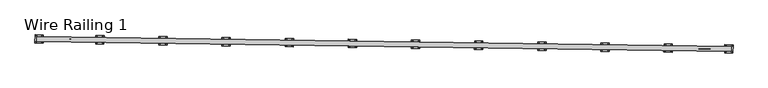
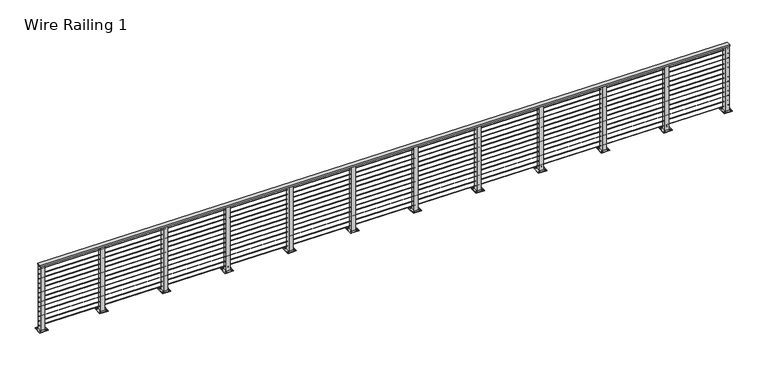
"""IFC4 building model written with IfcOpenShell, lengths in millimetres: railing geometry, Wire Railing 1."""

import ifcopenshell
import ifcopenshell.guid

model = None  # the IFC model being written
_history = None  # IfcOwnerHistory: only IFC2X3 demands one
_inside = {}  # id of a spatial element -> (the spatial element, [elements in it])
_under = {}  # id of a project, library or spatial element -> (it, [spatial elements below it])
_declared = {}  # id of a project -> (the project, [libraries it declares])
_typed = {}  # id of a type object -> (the type object, [elements of that type])
_made_of = {}  # id of a material, layer set ... -> (it, [elements and type objects made of it])


def new_model(schema):
    """Start an empty IFC model of exactly this schema.

    Asked for "IFC4X3", IfcOpenShell would pick the latest addendum, in which some entities
    have other attributes; the version numbers below select the first issue.
    IFC2X3 requires an IfcOwnerHistory on every rooted entity: one is made here for all.
    """
    global model, _history
    if schema == "IFC4X3":
        model = ifcopenshell.file(schema_version=(4, 3, 0, 0))
    else:
        model = ifcopenshell.file(schema=schema)
    _inside.clear()
    _under.clear()
    _declared.clear()
    _typed.clear()
    _made_of.clear()
    _history = None
    if model.schema == "IFC2X3":
        org = make("IfcOrganization", Name="unknown")
        user = make(
            "IfcPersonAndOrganization",
            ThePerson=make("IfcPerson", FamilyName="unknown"),
            TheOrganization=org,
        )
        app = make(
            "IfcApplication",
            ApplicationDeveloper=org,
            Version="unknown",
            ApplicationFullName="unknown",
            ApplicationIdentifier="unknown",
        )
        _history = make(
            "IfcOwnerHistory",
            OwningUser=user,
            OwningApplication=app,
            ChangeAction="ADDED",
            CreationDate=0,
        )
    return model


def make(cls, **values):
    """One entity of the class cls with the attributes given. An attribute that is None is left unset."""
    return model.create_entity(
        cls, **{name: value for name, value in values.items() if value is not None}
    )


def rooted(cls, **values):
    """An entity with a GlobalId (a new one), such as an element, a storey or a relation."""
    return make(cls, GlobalId=ifcopenshell.guid.new(), OwnerHistory=_history, **values)


def si_unit(unit_type, name, prefix=None):
    """IfcSIUnit, for example si_unit("LENGTHUNIT", "METRE", prefix="MILLI")."""
    return make("IfcSIUnit", UnitType=unit_type, Prefix=prefix, Name=name)


def assignment(units):
    """IfcUnitAssignment: the units of a project."""
    return None if units is None else make("IfcUnitAssignment", Units=units)


def point(xyz):
    """IfcCartesianPoint."""
    return None if xyz is None else make("IfcCartesianPoint", Coordinates=xyz)


def direction(xyz):
    """IfcDirection."""
    return None if xyz is None else make("IfcDirection", DirectionRatios=xyz)


def frame(location, z_axis=None, x_axis=None):
    """IfcAxis2Placement3D, a coordinate frame: its origin and axes. An axis left out is left unset."""
    return make(
        "IfcAxis2Placement3D",
        Location=point(location),
        Axis=direction(z_axis),
        RefDirection=direction(x_axis),
    )


def frame_2d(location, x_axis=None):
    """IfcAxis2Placement2D, a coordinate frame in the plane: its origin and x axis."""
    return make(
        "IfcAxis2Placement2D", Location=point(location), RefDirection=direction(x_axis)
    )


def origin():
    """The frame at (0, 0, 0) with its axes left unset."""
    return frame((0.0, 0.0, 0.0))


def place(relative_to, where):
    """IfcLocalPlacement: puts the frame where relative to a parent placement (None: the world)."""
    return make(
        "IfcLocalPlacement", PlacementRelTo=relative_to, RelativePlacement=where
    )


def context(
    kind, dimensions, precision=None, world=None, true_north=None, identifier=None
):
    """IfcGeometricRepresentationContext, for example the 3D "Model" context."""
    return make(
        "IfcGeometricRepresentationContext",
        ContextIdentifier=identifier,
        ContextType=kind,
        CoordinateSpaceDimension=dimensions,
        Precision=precision,
        WorldCoordinateSystem=world,
        TrueNorth=true_north,
    )


def project(units=None, contexts=None):
    """IfcProject with its units and contexts."""
    return rooted(
        "IfcProject",
        Name="project",
        RepresentationContexts=contexts,
        UnitsInContext=assignment(units),
    )


def spatial(cls, under=None, at=None, **own):
    """A site, building, storey or space (cls), placed at a placement, below another one or the project."""
    s = rooted(cls, ObjectPlacement=at, **own)
    if under is not None:
        _under.setdefault(under.id(), (under, []))[1].append(s)
    return s


def polyline(points):
    """IfcPolyline through the points."""
    return make("IfcPolyline", Points=[point(p) for p in points])


def circle_curve(where, radius):
    """IfcCircle in the frame where."""
    return make("IfcCircle", Position=where, Radius=radius)


def trimmed(basis, trim1, trim2, sense, master):
    """IfcTrimmedCurve: the piece of a basis curve between two trims."""
    return make(
        "IfcTrimmedCurve",
        BasisCurve=basis,
        Trim1=trim1,
        Trim2=trim2,
        SenseAgreement=sense,
        MasterRepresentation=master,
    )


def segment(curve, same_sense, transition):
    """IfcCompositeCurveSegment."""
    return make(
        "IfcCompositeCurveSegment",
        Transition=transition,
        SameSense=same_sense,
        ParentCurve=curve,
    )


def composite_curve(segments, self_intersect=None):
    """IfcCompositeCurve: segments joined end to end."""
    return make("IfcCompositeCurve", Segments=segments, SelfIntersect=self_intersect)


def outline(outer, holes=None, kind="AREA"):
    """IfcArbitraryClosedProfileDef: a profile drawn as a closed curve; with holes, ...WithVoids."""
    if holes is None:
        return make("IfcArbitraryClosedProfileDef", ProfileType=kind, OuterCurve=outer)
    return make(
        "IfcArbitraryProfileDefWithVoids",
        ProfileType=kind,
        OuterCurve=outer,
        InnerCurves=holes,
    )


def extrude(swept, where, along, depth):
    """IfcExtrudedAreaSolid: the profile swept, set in the frame where, extruded along a direction by depth."""
    return make(
        "IfcExtrudedAreaSolid",
        SweptArea=swept,
        Position=where,
        ExtrudedDirection=direction(along),
        Depth=depth,
    )


def shape(context_of_items, identifier, shape_type, items):
    """IfcShapeRepresentation: the items that make up one representation, for example the "Body"."""
    return make(
        "IfcShapeRepresentation",
        ContextOfItems=context_of_items,
        RepresentationIdentifier=identifier,
        RepresentationType=shape_type,
        Items=items,
    )


def source(mapping_origin, context_of_items, identifier, shape_type, items):
    """IfcRepresentationMap: a shape defined once, which mapped items show again and again."""
    return make(
        "IfcRepresentationMap",
        MappingOrigin=mapping_origin,
        MappedRepresentation=shape(context_of_items, identifier, shape_type, items),
    )


def transform(
    local_origin,
    x_axis=None,
    y_axis=None,
    z_axis=None,
    scale=None,
    scale2=None,
    scale3=None,
    uniform=True,
):
    """IfcCartesianTransformationOperator3D, or its non-uniform kind. x_axis, y_axis, z_axis: its Axis1, 2, 3."""
    if uniform:
        return make(
            "IfcCartesianTransformationOperator3D",
            Axis1=direction(x_axis),
            Axis2=direction(y_axis),
            LocalOrigin=point(local_origin),
            Scale=scale,
            Axis3=direction(z_axis),
        )
    return make(
        "IfcCartesianTransformationOperator3DnonUniform",
        Axis1=direction(x_axis),
        Axis2=direction(y_axis),
        LocalOrigin=point(local_origin),
        Scale=scale,
        Axis3=direction(z_axis),
        Scale2=scale2,
        Scale3=scale3,
    )


def mapped(mapping_source, mapping_target):
    """IfcMappedItem: shows the shape of a source again, moved by a transform."""
    return make(
        "IfcMappedItem", MappingSource=mapping_source, MappingTarget=mapping_target
    )


def made_of(thing, what):
    """Note that an element or type object is made of a material, layer set ...; save() writes the relation."""
    if what is not None:
        _made_of.setdefault(what.id(), (what, []))[1].append(thing)
    return thing


def element(
    cls,
    number,
    at=None,
    inside=None,
    cuts=None,
    type_object=None,
    material=None,
    context=None,
    identifier="Body",
    shape_type=None,
    held_by="IfcProductDefinitionShape",
    body=None,
    shapes=None,
    **own,
):
    """One element of the class cls, such as IfcWall. Its Tag is "e" and its number.

    at: its placement. inside: the storey or other place that contains it. cuts: it is an
    opening in that element (IfcRelVoidsElement). A single representation is given by context,
    identifier, shape_type and body (its items); several are given by shapes. held_by: the class
    of the entity that holds the representations. save() writes the other relations.
    """
    e = rooted(cls, Tag="e%d" % number, ObjectPlacement=at, **own)
    if body is not None:
        shapes = [shape(context, identifier, shape_type, body)]
    if shapes is not None:
        e.Representation = make(held_by, Representations=shapes)
    if inside is not None:
        _inside.setdefault(inside.id(), (inside, []))[1].append(e)
    if cuts is not None:
        rooted(
            "IfcRelVoidsElement", RelatingBuildingElement=cuts, RelatedOpeningElement=e
        )
    if type_object is not None:
        _typed.setdefault(type_object.id(), (type_object, []))[1].append(e)
    return made_of(e, material)


def aggregate(whole, parts):
    """IfcRelAggregates: a whole, such as a stair, and the parts it consists of."""
    return rooted("IfcRelAggregates", RelatingObject=whole, RelatedObjects=parts)


def save(model, path):
    """Write the relations noted so far, then the file.

    IfcRelAggregates (storeys below a building ...), IfcRelContainedInSpatialStructure (elements
    in a storey), IfcRelDefinesByType, IfcRelAssociatesMaterial and IfcRelDeclares: one each for
    every whole, place, type object, material and project.
    """
    for whole, parts in _under.values():
        aggregate(whole, parts)
    for where, things in _inside.values():
        rooted(
            "IfcRelContainedInSpatialStructure",
            RelatedElements=things,
            RelatingStructure=where,
        )
    for kind, things in _typed.values():
        rooted("IfcRelDefinesByType", RelatedObjects=things, RelatingType=kind)
    for what, things in _made_of.values():
        rooted("IfcRelAssociatesMaterial", RelatedObjects=things, RelatingMaterial=what)
    for by, libraries in _declared.values():
        rooted("IfcRelDeclares", RelatingContext=by, RelatedDefinitions=libraries)
    model.write(path)


def wire_railing_1_a902e167(model_context):
    return source(origin(), model_context, "Body", "SweptSolid", [
        extrude(outline(polyline([(35445.2454193, 41277.4063498), (35446.3492316, 41353.5983546), (45957.1135693, 41201.326324), (45956.009757, 41125.1343191), (35445.2454193, 41277.4063498)])), frame((0.0, 0.0, 267138.15), z_axis=(0.0, 0.0, 1.0), x_axis=(1.0, 0.0, 0.0)), (0.0, 0.0, 1.0), 19.05),
        extrude(outline(composite_curve([segment(trimmed(circle_curve(frame_2d((0.0, 2.38125)), 2.38125), [point((2.3812499, 2.38125))], [point((-2.3812501, 2.38125))], False, "CARTESIAN"), True, "CONTINUOUS"), segment(trimmed(circle_curve(frame_2d((0.0, 2.38125)), 2.38125), [point((-2.3812501, 2.38125))], [point((2.3812499, 2.38125))], False, "CARTESIAN"), True, "CONTINUOUS")], self_intersect=False)), frame((45956.5616632, 41163.2303216, 267081.0), z_axis=(-0.9998950763646337, 0.014485726138629394, 0.0), x_axis=(0.014485726138629394, 0.9998950763646337, 0.0)), (0.0, 0.0, 1.0), 10511.8672811),
        extrude(outline(composite_curve([segment(trimmed(circle_curve(frame_2d((0.0, 2.38125)), 2.38125), [point((2.3812499, 2.38125))], [point((-2.3812501, 2.38125))], False, "CARTESIAN"), True, "CONTINUOUS"), segment(trimmed(circle_curve(frame_2d((0.0, 2.38125)), 2.38125), [point((-2.3812501, 2.38125))], [point((2.3812499, 2.38125))], False, "CARTESIAN"), True, "CONTINUOUS")], self_intersect=False)), frame((45956.5616632, 41163.2303216, 267004.8), z_axis=(-0.9998950763646337, 0.014485726138629394, 0.0), x_axis=(0.014485726138629394, 0.9998950763646337, 0.0)), (0.0, 0.0, 1.0), 10511.8672811),
        extrude(outline(composite_curve([segment(trimmed(circle_curve(frame_2d((0.0, 2.38125)), 2.38125), [point((2.3812499, 2.38125))], [point((-2.3812501, 2.38125))], False, "CARTESIAN"), True, "CONTINUOUS"), segment(trimmed(circle_curve(frame_2d((0.0, 2.38125)), 2.38125), [point((-2.3812501, 2.38125))], [point((2.3812499, 2.38125))], False, "CARTESIAN"), True, "CONTINUOUS")], self_intersect=False)), frame((45956.5616632, 41163.2303216, 266928.6), z_axis=(-0.9998950763646337, 0.014485726138629394, 0.0), x_axis=(0.014485726138629394, 0.9998950763646337, 0.0)), (0.0, 0.0, 1.0), 10511.8672811),
        extrude(outline(composite_curve([segment(trimmed(circle_curve(frame_2d((0.0, 2.38125)), 2.38125), [point((2.3812499, 2.38125))], [point((-2.3812501, 2.38125))], False, "CARTESIAN"), True, "CONTINUOUS"), segment(trimmed(circle_curve(frame_2d((0.0, 2.38125)), 2.38125), [point((-2.3812501, 2.38125))], [point((2.3812499, 2.38125))], False, "CARTESIAN"), True, "CONTINUOUS")], self_intersect=False)), frame((45956.5616632, 41163.2303216, 266852.4), z_axis=(-0.9998950763646337, 0.014485726138629394, 0.0), x_axis=(0.014485726138629394, 0.9998950763646337, 0.0)), (0.0, 0.0, 1.0), 10511.8672811),
        extrude(outline(composite_curve([segment(trimmed(circle_curve(frame_2d((0.0, 2.38125)), 2.38125), [point((2.3812499, 2.38125))], [point((-2.3812501, 2.38125))], False, "CARTESIAN"), True, "CONTINUOUS"), segment(trimmed(circle_curve(frame_2d((0.0, 2.38125)), 2.38125), [point((-2.3812501, 2.38125))], [point((2.3812499, 2.38125))], False, "CARTESIAN"), True, "CONTINUOUS")], self_intersect=False)), frame((45956.5616632, 41163.2303216, 266776.2), z_axis=(-0.9998950763646337, 0.014485726138629394, 0.0), x_axis=(0.014485726138629394, 0.9998950763646337, 0.0)), (0.0, 0.0, 1.0), 10511.8672811),
        extrude(outline(composite_curve([segment(trimmed(circle_curve(frame_2d((0.0, 2.38125)), 2.38125), [point((2.3812499, 2.38125))], [point((-2.3812501, 2.38125))], False, "CARTESIAN"), True, "CONTINUOUS"), segment(trimmed(circle_curve(frame_2d((0.0, 2.38125)), 2.38125), [point((-2.3812501, 2.38125))], [point((2.3812499, 2.38125))], False, "CARTESIAN"), True, "CONTINUOUS")], self_intersect=False)), frame((45956.5616632, 41163.2303216, 266700.0), z_axis=(-0.9998950763646337, 0.014485726138629394, 0.0), x_axis=(0.014485726138629394, 0.9998950763646337, 0.0)), (0.0, 0.0, 1.0), 10511.8672811),
        extrude(outline(composite_curve([segment(trimmed(circle_curve(frame_2d((0.0, 2.38125)), 2.38125), [point((2.3812499, 2.38125))], [point((-2.3812501, 2.38125))], False, "CARTESIAN"), True, "CONTINUOUS"), segment(trimmed(circle_curve(frame_2d((0.0, 2.38125)), 2.38125), [point((-2.3812501, 2.38125))], [point((2.3812499, 2.38125))], False, "CARTESIAN"), True, "CONTINUOUS")], self_intersect=False)), frame((45956.5616632, 41163.2303216, 266623.8), z_axis=(-0.9998950763646337, 0.014485726138629394, 0.0), x_axis=(0.014485726138629394, 0.9998950763646337, 0.0)), (0.0, 0.0, 1.0), 10511.8672811),
        extrude(outline(composite_curve([segment(trimmed(circle_curve(frame_2d((0.0, 2.38125)), 2.38125), [point((2.3812499, 2.38125))], [point((-2.3812501, 2.38125))], False, "CARTESIAN"), True, "CONTINUOUS"), segment(trimmed(circle_curve(frame_2d((0.0, 2.38125)), 2.38125), [point((-2.3812501, 2.38125))], [point((2.3812499, 2.38125))], False, "CARTESIAN"), True, "CONTINUOUS")], self_intersect=False)), frame((45956.5616632, 41163.2303216, 266547.6), z_axis=(-0.9998950763646337, 0.014485726138629394, 0.0), x_axis=(0.014485726138629394, 0.9998950763646337, 0.0)), (0.0, 0.0, 1.0), 10511.8672811),
        extrude(outline(composite_curve([segment(trimmed(circle_curve(frame_2d((0.0, 2.38125)), 2.38125), [point((2.3812499, 2.38125))], [point((-2.3812501, 2.38125))], False, "CARTESIAN"), True, "CONTINUOUS"), segment(trimmed(circle_curve(frame_2d((0.0, 2.38125)), 2.38125), [point((-2.3812501, 2.38125))], [point((2.3812499, 2.38125))], False, "CARTESIAN"), True, "CONTINUOUS")], self_intersect=False)), frame((45956.5616632, 41163.2303216, 266471.4), z_axis=(-0.9998950763646337, 0.014485726138629394, 0.0), x_axis=(0.014485726138629394, 0.9998950763646337, 0.0)), (0.0, 0.0, 1.0), 10511.8672811),
        extrude(outline(composite_curve([segment(trimmed(circle_curve(frame_2d((0.0, 2.38125)), 2.38125), [point((2.3812499, 2.38125))], [point((-2.3812501, 2.38125))], False, "CARTESIAN"), True, "CONTINUOUS"), segment(trimmed(circle_curve(frame_2d((0.0, 2.38125)), 2.38125), [point((-2.3812501, 2.38125))], [point((2.3812499, 2.38125))], False, "CARTESIAN"), True, "CONTINUOUS")], self_intersect=False)), frame((45956.5616632, 41163.2303216, 266395.2), z_axis=(-0.9998950763646337, 0.014485726138629394, 0.0), x_axis=(0.014485726138629394, 0.9998950763646337, 0.0)), (0.0, 0.0, 1.0), 10511.8672811),
        extrude(outline(composite_curve([segment(trimmed(circle_curve(frame_2d((0.0, 2.38125)), 2.38125), [point((2.3812499, 2.38125))], [point((-2.3812501, 2.38125))], False, "CARTESIAN"), True, "CONTINUOUS"), segment(trimmed(circle_curve(frame_2d((0.0, 2.38125)), 2.38125), [point((-2.3812501, 2.38125))], [point((2.3812499, 2.38125))], False, "CARTESIAN"), True, "CONTINUOUS")], self_intersect=False)), frame((45956.5616632, 41163.2303216, 266319.0), z_axis=(-0.9998950763646337, 0.014485726138629394, 0.0), x_axis=(0.014485726138629394, 0.9998950763646337, 0.0)), (0.0, 0.0, 1.0), 10511.8672811),
        extrude(outline(composite_curve([segment(trimmed(circle_curve(frame_2d((0.0, 2.38125)), 2.38125), [point((2.3812499, 2.38125))], [point((-2.3812501, 2.38125))], False, "CARTESIAN"), True, "CONTINUOUS"), segment(trimmed(circle_curve(frame_2d((0.0, 2.38125)), 2.38125), [point((-2.3812501, 2.38125))], [point((2.3812499, 2.38125))], False, "CARTESIAN"), True, "CONTINUOUS")], self_intersect=False)), frame((45956.5616632, 41163.2303216, 266242.8), z_axis=(-0.9998950763646337, 0.014485726138629394, 0.0), x_axis=(0.014485726138629394, 0.9998950763646337, 0.0)), (0.0, 0.0, 1.0), 10511.8672811),
        extrude(outline(composite_curve([segment(trimmed(circle_curve(frame_2d((0.0, 2.38125)), 2.38125), [point((2.3812499, 2.38125))], [point((-2.3812501, 2.38125))], False, "CARTESIAN"), True, "CONTINUOUS"), segment(trimmed(circle_curve(frame_2d((0.0, 2.38125)), 2.38125), [point((-2.3812501, 2.38125))], [point((2.3812499, 2.38125))], False, "CARTESIAN"), True, "CONTINUOUS")], self_intersect=False)), frame((45956.5616632, 41163.2303216, 266166.6), z_axis=(-0.9998950763646337, 0.014485726138629394, 0.0), x_axis=(0.014485726138629394, 0.9998950763646337, 0.0)), (0.0, 0.0, 1.0), 10511.8672811),
        extrude(outline(composite_curve([segment(trimmed(circle_curve(frame_2d((44955.9484058, 41133.2717878)), 6.35), [point((44955.8564214, 41126.9224541))], [point((44956.0403902, 41139.6211215))], False, "CARTESIAN"), True, "CONTINUOUS"), segment(trimmed(circle_curve(frame_2d((44955.9484058, 41133.2717878)), 6.35), [point((44956.0403902, 41139.6211215))], [point((44955.8564214, 41126.9224541))], False, "CARTESIAN"), True, "CONTINUOUS")], self_intersect=False)), frame((0.0, 0.0, 266090.4), z_axis=(0.0, 0.0, 1.0), x_axis=(1.0, 0.0, 0.0)), (0.0, 0.0, 1.0), 12.7),
        extrude(outline(composite_curve([segment(trimmed(circle_curve(frame_2d((44957.2361869, 41222.1624601)), 6.35), [point((44957.1442025, 41215.8131264))], [point((44957.3281712, 41228.5117938))], False, "CARTESIAN"), True, "CONTINUOUS"), segment(trimmed(circle_curve(frame_2d((44957.2361869, 41222.1624601)), 6.35), [point((44957.3281712, 41228.5117938))], [point((44957.1442025, 41215.8131264))], False, "CARTESIAN"), True, "CONTINUOUS")], self_intersect=False)), frame((0.0, 0.0, 266090.4), z_axis=(0.0, 0.0, 1.0), x_axis=(1.0, 0.0, 0.0)), (0.0, 0.0, 1.0), 12.7),
        extrude(outline(composite_curve([segment(trimmed(circle_curve(frame_2d((45044.8390781, 41131.9840068)), 6.35), [point((45044.7470937, 41125.634673))], [point((45044.9310624, 41138.3333405))], False, "CARTESIAN"), True, "CONTINUOUS"), segment(trimmed(circle_curve(frame_2d((45044.8390781, 41131.9840068)), 6.35), [point((45044.9310624, 41138.3333405))], [point((45044.7470937, 41125.634673))], False, "CARTESIAN"), True, "CONTINUOUS")], self_intersect=False)), frame((0.0, 0.0, 266090.4), z_axis=(0.0, 0.0, 1.0), x_axis=(1.0, 0.0, 0.0)), (0.0, 0.0, 1.0), 12.7),
        extrude(outline(composite_curve([segment(trimmed(circle_curve(frame_2d((45046.1268591, 41220.874679)), 6.35), [point((45046.0348748, 41214.5253453))], [point((45046.2188435, 41227.2240128))], False, "CARTESIAN"), True, "CONTINUOUS"), segment(trimmed(circle_curve(frame_2d((45046.1268591, 41220.874679)), 6.35), [point((45046.2188435, 41227.2240128))], [point((45046.0348748, 41214.5253453))], False, "CARTESIAN"), True, "CONTINUOUS")], self_intersect=False)), frame((0.0, 0.0, 266090.4), z_axis=(0.0, 0.0, 1.0), x_axis=(1.0, 0.0, 0.0)), (0.0, 0.0, 1.0), 12.7),
        extrude(outline(polyline([(44938.4641387, 41241.4864144), (45065.4508134, 41239.6467272), (45063.6111262, 41112.6600525), (44936.6244515, 41114.4997397), (44938.4641387, 41241.4864144)])), frame((0.0, 0.0, 266090.4), z_axis=(0.0, 0.0, 1.0), x_axis=(1.0, 0.0, 0.0)), (0.0, 0.0, 1.0), 6.35),
        extrude(outline(polyline([(44971.3152229, 41207.6694944), (45031.6338934, 41206.795643), (45030.760042, 41146.4769725), (44970.4413715, 41147.3508239), (44971.3152229, 41207.6694944)]), holes=[polyline([(44977.5725723, 41201.2281763), (44976.8826896, 41153.6081733), (45024.5026926, 41152.9182906), (45025.1925753, 41200.5382936), (44977.5725723, 41201.2281763)])]), frame((0.0, 0.0, 266090.4), z_axis=(0.0, 0.0, 1.0), x_axis=(1.0, 0.0, 0.0)), (0.0, 0.0, 1.0), 1047.75),
        extrude(outline(composite_curve([segment(trimmed(circle_curve(frame_2d((44000.4243751, 41147.1146997)), 6.35), [point((44000.3323907, 41140.765366))], [point((44000.5163595, 41153.4640334))], False, "CARTESIAN"), True, "CONTINUOUS"), segment(trimmed(circle_curve(frame_2d((44000.4243751, 41147.1146997)), 6.35), [point((44000.5163595, 41153.4640334))], [point((44000.3323907, 41140.765366))], False, "CARTESIAN"), True, "CONTINUOUS")], self_intersect=False)), frame((0.0, 0.0, 266090.4), z_axis=(0.0, 0.0, 1.0), x_axis=(1.0, 0.0, 0.0)), (0.0, 0.0, 1.0), 12.7),
        extrude(outline(composite_curve([segment(trimmed(circle_curve(frame_2d((44001.7121561, 41236.005372)), 6.35), [point((44001.6201718, 41229.6560382))], [point((44001.8041405, 41242.3547057))], False, "CARTESIAN"), True, "CONTINUOUS"), segment(trimmed(circle_curve(frame_2d((44001.7121561, 41236.005372)), 6.35), [point((44001.8041405, 41242.3547057))], [point((44001.6201718, 41229.6560382))], False, "CARTESIAN"), True, "CONTINUOUS")], self_intersect=False)), frame((0.0, 0.0, 266090.4), z_axis=(0.0, 0.0, 1.0), x_axis=(1.0, 0.0, 0.0)), (0.0, 0.0, 1.0), 12.7),
        extrude(outline(composite_curve([segment(trimmed(circle_curve(frame_2d((44089.3150474, 41145.8269186)), 6.35), [point((44089.223063, 41139.4775849))], [point((44089.4070317, 41152.1762524))], False, "CARTESIAN"), True, "CONTINUOUS"), segment(trimmed(circle_curve(frame_2d((44089.3150474, 41145.8269186)), 6.35), [point((44089.4070317, 41152.1762524))], [point((44089.223063, 41139.4775849))], False, "CARTESIAN"), True, "CONTINUOUS")], self_intersect=False)), frame((0.0, 0.0, 266090.4), z_axis=(0.0, 0.0, 1.0), x_axis=(1.0, 0.0, 0.0)), (0.0, 0.0, 1.0), 12.7),
        extrude(outline(composite_curve([segment(trimmed(circle_curve(frame_2d((44090.6028284, 41234.7175909)), 6.35), [point((44090.5108441, 41228.3682572))], [point((44090.6948128, 41241.0669247))], False, "CARTESIAN"), True, "CONTINUOUS"), segment(trimmed(circle_curve(frame_2d((44090.6028284, 41234.7175909)), 6.35), [point((44090.6948128, 41241.0669247))], [point((44090.5108441, 41228.3682572))], False, "CARTESIAN"), True, "CONTINUOUS")], self_intersect=False)), frame((0.0, 0.0, 266090.4), z_axis=(0.0, 0.0, 1.0), x_axis=(1.0, 0.0, 0.0)), (0.0, 0.0, 1.0), 12.7),
        extrude(outline(polyline([(43982.940108, 41255.3293263), (44109.9267827, 41253.489639), (44108.0870955, 41126.5029643), (43981.1004208, 41128.3426516), (43982.940108, 41255.3293263)])), frame((0.0, 0.0, 266090.4), z_axis=(0.0, 0.0, 1.0), x_axis=(1.0, 0.0, 0.0)), (0.0, 0.0, 1.0), 6.35),
        extrude(outline(polyline([(44015.7911922, 41221.5124063), (44076.1098627, 41220.6385548), (44075.2360113, 41160.3198844), (44014.9173408, 41161.1937358), (44015.7911922, 41221.5124063)]), holes=[polyline([(44022.0485416, 41215.0710882), (44021.3586589, 41167.4510852), (44068.9786619, 41166.7612024), (44069.6685446, 41214.3812055), (44022.0485416, 41215.0710882)])]), frame((0.0, 0.0, 266090.4), z_axis=(0.0, 0.0, 1.0), x_axis=(1.0, 0.0, 0.0)), (0.0, 0.0, 1.0), 1047.75),
        extrude(outline(composite_curve([segment(trimmed(circle_curve(frame_2d((43044.9003444, 41160.9576116)), 6.35), [point((43044.80836, 41154.6082778))], [point((43044.9923287, 41167.3069453))], False, "CARTESIAN"), True, "CONTINUOUS"), segment(trimmed(circle_curve(frame_2d((43044.9003444, 41160.9576116)), 6.35), [point((43044.9923287, 41167.3069453))], [point((43044.80836, 41154.6082778))], False, "CARTESIAN"), True, "CONTINUOUS")], self_intersect=False)), frame((0.0, 0.0, 266090.4), z_axis=(0.0, 0.0, 1.0), x_axis=(1.0, 0.0, 0.0)), (0.0, 0.0, 1.0), 12.7),
        extrude(outline(composite_curve([segment(trimmed(circle_curve(frame_2d((43046.1881254, 41249.8482839)), 6.35), [point((43046.0961411, 41243.4989501))], [point((43046.2801098, 41256.1976176))], False, "CARTESIAN"), True, "CONTINUOUS"), segment(trimmed(circle_curve(frame_2d((43046.1881254, 41249.8482839)), 6.35), [point((43046.2801098, 41256.1976176))], [point((43046.0961411, 41243.4989501))], False, "CARTESIAN"), True, "CONTINUOUS")], self_intersect=False)), frame((0.0, 0.0, 266090.4), z_axis=(0.0, 0.0, 1.0), x_axis=(1.0, 0.0, 0.0)), (0.0, 0.0, 1.0), 12.7),
        extrude(outline(composite_curve([segment(trimmed(circle_curve(frame_2d((43133.7910167, 41159.6698305)), 6.35), [point((43133.6990323, 41153.3204968))], [point((43133.883001, 41166.0191642))], False, "CARTESIAN"), True, "CONTINUOUS"), segment(trimmed(circle_curve(frame_2d((43133.7910167, 41159.6698305)), 6.35), [point((43133.883001, 41166.0191642))], [point((43133.6990323, 41153.3204968))], False, "CARTESIAN"), True, "CONTINUOUS")], self_intersect=False)), frame((0.0, 0.0, 266090.4), z_axis=(0.0, 0.0, 1.0), x_axis=(1.0, 0.0, 0.0)), (0.0, 0.0, 1.0), 12.7),
        extrude(outline(composite_curve([segment(trimmed(circle_curve(frame_2d((43135.0787977, 41248.5605028)), 6.35), [point((43134.9868134, 41242.2111691))], [point((43135.1707821, 41254.9098365))], False, "CARTESIAN"), True, "CONTINUOUS"), segment(trimmed(circle_curve(frame_2d((43135.0787977, 41248.5605028)), 6.35), [point((43135.1707821, 41254.9098365))], [point((43134.9868134, 41242.2111691))], False, "CARTESIAN"), True, "CONTINUOUS")], self_intersect=False)), frame((0.0, 0.0, 266090.4), z_axis=(0.0, 0.0, 1.0), x_axis=(1.0, 0.0, 0.0)), (0.0, 0.0, 1.0), 12.7),
        extrude(outline(polyline([(43027.4160773, 41269.1722381), (43154.402752, 41267.3325509), (43152.5630648, 41140.3458762), (43025.5763901, 41142.1855634), (43027.4160773, 41269.1722381)])), frame((0.0, 0.0, 266090.4), z_axis=(0.0, 0.0, 1.0), x_axis=(1.0, 0.0, 0.0)), (0.0, 0.0, 1.0), 6.35),
        extrude(outline(polyline([(43060.2671615, 41235.3553181), (43120.585832, 41234.4814667), (43119.7119806, 41174.1627962), (43059.3933101, 41175.0366477), (43060.2671615, 41235.3553181)]), holes=[polyline([(43066.5245109, 41228.914), (43065.8346282, 41181.293997), (43113.4546312, 41180.6041143), (43114.1445139, 41228.2241173), (43066.5245109, 41228.914)])]), frame((0.0, 0.0, 266090.4), z_axis=(0.0, 0.0, 1.0), x_axis=(1.0, 0.0, 0.0)), (0.0, 0.0, 1.0), 1047.75),
        extrude(outline(composite_curve([segment(trimmed(circle_curve(frame_2d((42089.3763137, 41174.8005234)), 6.35), [point((42089.2843293, 41168.4511897))], [point((42089.468298, 41181.1498572))], False, "CARTESIAN"), True, "CONTINUOUS"), segment(trimmed(circle_curve(frame_2d((42089.3763137, 41174.8005234)), 6.35), [point((42089.468298, 41181.1498572))], [point((42089.2843293, 41168.4511897))], False, "CARTESIAN"), True, "CONTINUOUS")], self_intersect=False)), frame((0.0, 0.0, 266090.4), z_axis=(0.0, 0.0, 1.0), x_axis=(1.0, 0.0, 0.0)), (0.0, 0.0, 1.0), 12.7),
        extrude(outline(composite_curve([segment(trimmed(circle_curve(frame_2d((42090.6640947, 41263.6911957)), 6.35), [point((42090.5721104, 41257.341862))], [point((42090.7560791, 41270.0405295))], False, "CARTESIAN"), True, "CONTINUOUS"), segment(trimmed(circle_curve(frame_2d((42090.6640947, 41263.6911957)), 6.35), [point((42090.7560791, 41270.0405295))], [point((42090.5721104, 41257.341862))], False, "CARTESIAN"), True, "CONTINUOUS")], self_intersect=False)), frame((0.0, 0.0, 266090.4), z_axis=(0.0, 0.0, 1.0), x_axis=(1.0, 0.0, 0.0)), (0.0, 0.0, 1.0), 12.7),
        extrude(outline(composite_curve([segment(trimmed(circle_curve(frame_2d((42178.266986, 41173.5127424)), 6.35), [point((42178.1750016, 41167.1634087))], [point((42178.3589703, 41179.8620761))], False, "CARTESIAN"), True, "CONTINUOUS"), segment(trimmed(circle_curve(frame_2d((42178.266986, 41173.5127424)), 6.35), [point((42178.3589703, 41179.8620761))], [point((42178.1750016, 41167.1634087))], False, "CARTESIAN"), True, "CONTINUOUS")], self_intersect=False)), frame((0.0, 0.0, 266090.4), z_axis=(0.0, 0.0, 1.0), x_axis=(1.0, 0.0, 0.0)), (0.0, 0.0, 1.0), 12.7),
        extrude(outline(composite_curve([segment(trimmed(circle_curve(frame_2d((42179.554767, 41262.4034147)), 6.35), [point((42179.4627827, 41256.0540809))], [point((42179.6467514, 41268.7527484))], False, "CARTESIAN"), True, "CONTINUOUS"), segment(trimmed(circle_curve(frame_2d((42179.554767, 41262.4034147)), 6.35), [point((42179.6467514, 41268.7527484))], [point((42179.4627827, 41256.0540809))], False, "CARTESIAN"), True, "CONTINUOUS")], self_intersect=False)), frame((0.0, 0.0, 266090.4), z_axis=(0.0, 0.0, 1.0), x_axis=(1.0, 0.0, 0.0)), (0.0, 0.0, 1.0), 12.7),
        extrude(outline(polyline([(42071.8920466, 41283.01515), (42198.8787213, 41281.1754628), (42197.0390341, 41154.1887881), (42070.0523594, 41156.0284753), (42071.8920466, 41283.01515)])), frame((0.0, 0.0, 266090.4), z_axis=(0.0, 0.0, 1.0), x_axis=(1.0, 0.0, 0.0)), (0.0, 0.0, 1.0), 6.35),
        extrude(outline(polyline([(42104.7431308, 41249.19823), (42165.0618013, 41248.3243786), (42164.1879499, 41188.0057081), (42103.8692794, 41188.8795595), (42104.7431308, 41249.19823)]), holes=[polyline([(42111.0004802, 41242.7569119), (42110.3105975, 41195.1369089), (42157.9306005, 41194.4470262), (42158.6204832, 41242.0670292), (42111.0004802, 41242.7569119)])]), frame((0.0, 0.0, 266090.4), z_axis=(0.0, 0.0, 1.0), x_axis=(1.0, 0.0, 0.0)), (0.0, 0.0, 1.0), 1047.75),
        extrude(outline(composite_curve([segment(trimmed(circle_curve(frame_2d((41133.852283, 41188.6434353)), 6.35), [point((41133.7602986, 41182.2941016))], [point((41133.9442673, 41194.9927691))], False, "CARTESIAN"), True, "CONTINUOUS"), segment(trimmed(circle_curve(frame_2d((41133.852283, 41188.6434353)), 6.35), [point((41133.9442673, 41194.9927691))], [point((41133.7602986, 41182.2941016))], False, "CARTESIAN"), True, "CONTINUOUS")], self_intersect=False)), frame((0.0, 0.0, 266090.4), z_axis=(0.0, 0.0, 1.0), x_axis=(1.0, 0.0, 0.0)), (0.0, 0.0, 1.0), 12.7),
        extrude(outline(composite_curve([segment(trimmed(circle_curve(frame_2d((41135.140064, 41277.5341076)), 6.35), [point((41135.0480797, 41271.1847739))], [point((41135.2320484, 41283.8834413))], False, "CARTESIAN"), True, "CONTINUOUS"), segment(trimmed(circle_curve(frame_2d((41135.140064, 41277.5341076)), 6.35), [point((41135.2320484, 41283.8834413))], [point((41135.0480797, 41271.1847739))], False, "CARTESIAN"), True, "CONTINUOUS")], self_intersect=False)), frame((0.0, 0.0, 266090.4), z_axis=(0.0, 0.0, 1.0), x_axis=(1.0, 0.0, 0.0)), (0.0, 0.0, 1.0), 12.7),
        extrude(outline(composite_curve([segment(trimmed(circle_curve(frame_2d((41222.7429553, 41187.3556543)), 6.35), [point((41222.6509709, 41181.0063205))], [point((41222.8349396, 41193.704988))], False, "CARTESIAN"), True, "CONTINUOUS"), segment(trimmed(circle_curve(frame_2d((41222.7429553, 41187.3556543)), 6.35), [point((41222.8349396, 41193.704988))], [point((41222.6509709, 41181.0063205))], False, "CARTESIAN"), True, "CONTINUOUS")], self_intersect=False)), frame((0.0, 0.0, 266090.4), z_axis=(0.0, 0.0, 1.0), x_axis=(1.0, 0.0, 0.0)), (0.0, 0.0, 1.0), 12.7),
        extrude(outline(composite_curve([segment(trimmed(circle_curve(frame_2d((41224.0307363, 41276.2463266)), 6.35), [point((41223.938752, 41269.8969928))], [point((41224.1227207, 41282.5956603))], False, "CARTESIAN"), True, "CONTINUOUS"), segment(trimmed(circle_curve(frame_2d((41224.0307363, 41276.2463266)), 6.35), [point((41224.1227207, 41282.5956603))], [point((41223.938752, 41269.8969928))], False, "CARTESIAN"), True, "CONTINUOUS")], self_intersect=False)), frame((0.0, 0.0, 266090.4), z_axis=(0.0, 0.0, 1.0), x_axis=(1.0, 0.0, 0.0)), (0.0, 0.0, 1.0), 12.7),
        extrude(outline(polyline([(41116.3680159, 41296.8580619), (41243.3546906, 41295.0183747), (41241.5150034, 41168.0317), (41114.5283287, 41169.8713872), (41116.3680159, 41296.8580619)])), frame((0.0, 0.0, 266090.4), z_axis=(0.0, 0.0, 1.0), x_axis=(1.0, 0.0, 0.0)), (0.0, 0.0, 1.0), 6.35),
        extrude(outline(polyline([(41149.2191001, 41263.0411419), (41209.5377706, 41262.1672905), (41208.6639192, 41201.84862), (41148.3452487, 41202.7224714), (41149.2191001, 41263.0411419)]), holes=[polyline([(41155.4764495, 41256.5998238), (41154.7865668, 41208.9798208), (41202.4065698, 41208.2899381), (41203.0964525, 41255.9099411), (41155.4764495, 41256.5998238)])]), frame((0.0, 0.0, 266090.4), z_axis=(0.0, 0.0, 1.0), x_axis=(1.0, 0.0, 0.0)), (0.0, 0.0, 1.0), 1047.75),
        extrude(outline(composite_curve([segment(trimmed(circle_curve(frame_2d((40178.3282523, 41202.4863472)), 6.35), [point((40178.2362679, 41196.1370135))], [point((40178.4202366, 41208.8356809))], False, "CARTESIAN"), True, "CONTINUOUS"), segment(trimmed(circle_curve(frame_2d((40178.3282523, 41202.4863472)), 6.35), [point((40178.4202366, 41208.8356809))], [point((40178.2362679, 41196.1370135))], False, "CARTESIAN"), True, "CONTINUOUS")], self_intersect=False)), frame((0.0, 0.0, 266090.4), z_axis=(0.0, 0.0, 1.0), x_axis=(1.0, 0.0, 0.0)), (0.0, 0.0, 1.0), 12.7),
        extrude(outline(composite_curve([segment(trimmed(circle_curve(frame_2d((40179.6160333, 41291.3770195)), 6.35), [point((40179.524049, 41285.0276857))], [point((40179.7080177, 41297.7263532))], False, "CARTESIAN"), True, "CONTINUOUS"), segment(trimmed(circle_curve(frame_2d((40179.6160333, 41291.3770195)), 6.35), [point((40179.7080177, 41297.7263532))], [point((40179.524049, 41285.0276857))], False, "CARTESIAN"), True, "CONTINUOUS")], self_intersect=False)), frame((0.0, 0.0, 266090.4), z_axis=(0.0, 0.0, 1.0), x_axis=(1.0, 0.0, 0.0)), (0.0, 0.0, 1.0), 12.7),
        extrude(outline(composite_curve([segment(trimmed(circle_curve(frame_2d((40267.2189246, 41201.1985661)), 6.35), [point((40267.1269402, 41194.8492324))], [point((40267.3109089, 41207.5478999))], False, "CARTESIAN"), True, "CONTINUOUS"), segment(trimmed(circle_curve(frame_2d((40267.2189246, 41201.1985661)), 6.35), [point((40267.3109089, 41207.5478999))], [point((40267.1269402, 41194.8492324))], False, "CARTESIAN"), True, "CONTINUOUS")], self_intersect=False)), frame((0.0, 0.0, 266090.4), z_axis=(0.0, 0.0, 1.0), x_axis=(1.0, 0.0, 0.0)), (0.0, 0.0, 1.0), 12.7),
        extrude(outline(composite_curve([segment(trimmed(circle_curve(frame_2d((40268.5067056, 41290.0892384)), 6.35), [point((40268.4147213, 41283.7399047))], [point((40268.59869, 41296.4385722))], False, "CARTESIAN"), True, "CONTINUOUS"), segment(trimmed(circle_curve(frame_2d((40268.5067056, 41290.0892384)), 6.35), [point((40268.59869, 41296.4385722))], [point((40268.4147213, 41283.7399047))], False, "CARTESIAN"), True, "CONTINUOUS")], self_intersect=False)), frame((0.0, 0.0, 266090.4), z_axis=(0.0, 0.0, 1.0), x_axis=(1.0, 0.0, 0.0)), (0.0, 0.0, 1.0), 12.7),
        extrude(outline(polyline([(40160.8439852, 41310.7009738), (40287.8306599, 41308.8612866), (40285.9909727, 41181.8746119), (40159.004298, 41183.7142991), (40160.8439852, 41310.7009738)])), frame((0.0, 0.0, 266090.4), z_axis=(0.0, 0.0, 1.0), x_axis=(1.0, 0.0, 0.0)), (0.0, 0.0, 1.0), 6.35),
        extrude(outline(polyline([(40193.6950694, 41276.8840538), (40254.0137399, 41276.0102023), (40253.1398885, 41215.6915319), (40192.821218, 41216.5653833), (40193.6950694, 41276.8840538)]), holes=[polyline([(40199.9524188, 41270.4427357), (40199.2625361, 41222.8227327), (40246.8825391, 41222.13285), (40247.5724218, 41269.752853), (40199.9524188, 41270.4427357)])]), frame((0.0, 0.0, 266090.4), z_axis=(0.0, 0.0, 1.0), x_axis=(1.0, 0.0, 0.0)), (0.0, 0.0, 1.0), 1047.75),
        extrude(outline(composite_curve([segment(trimmed(circle_curve(frame_2d((39222.8042216, 41216.3292591)), 6.35), [point((39222.7122372, 41209.9799253))], [point((39222.8962059, 41222.6785928))], False, "CARTESIAN"), True, "CONTINUOUS"), segment(trimmed(circle_curve(frame_2d((39222.8042216, 41216.3292591)), 6.35), [point((39222.8962059, 41222.6785928))], [point((39222.7122372, 41209.9799253))], False, "CARTESIAN"), True, "CONTINUOUS")], self_intersect=False)), frame((0.0, 0.0, 266090.4), z_axis=(0.0, 0.0, 1.0), x_axis=(1.0, 0.0, 0.0)), (0.0, 0.0, 1.0), 12.7),
        extrude(outline(composite_curve([segment(trimmed(circle_curve(frame_2d((39224.0920026, 41305.2199314)), 6.35), [point((39224.0000183, 41298.8705976))], [point((39224.183987, 41311.5692651))], False, "CARTESIAN"), True, "CONTINUOUS"), segment(trimmed(circle_curve(frame_2d((39224.0920026, 41305.2199314)), 6.35), [point((39224.183987, 41311.5692651))], [point((39224.0000183, 41298.8705976))], False, "CARTESIAN"), True, "CONTINUOUS")], self_intersect=False)), frame((0.0, 0.0, 266090.4), z_axis=(0.0, 0.0, 1.0), x_axis=(1.0, 0.0, 0.0)), (0.0, 0.0, 1.0), 12.7),
        extrude(outline(composite_curve([segment(trimmed(circle_curve(frame_2d((39311.6948939, 41215.041478)), 6.35), [point((39311.6029095, 41208.6921443))], [point((39311.7868782, 41221.3908118))], False, "CARTESIAN"), True, "CONTINUOUS"), segment(trimmed(circle_curve(frame_2d((39311.6948939, 41215.041478)), 6.35), [point((39311.7868782, 41221.3908118))], [point((39311.6029095, 41208.6921443))], False, "CARTESIAN"), True, "CONTINUOUS")], self_intersect=False)), frame((0.0, 0.0, 266090.4), z_axis=(0.0, 0.0, 1.0), x_axis=(1.0, 0.0, 0.0)), (0.0, 0.0, 1.0), 12.7),
        extrude(outline(composite_curve([segment(trimmed(circle_curve(frame_2d((39312.9826749, 41303.9321503)), 6.35), [point((39312.8906905, 41297.5828166))], [point((39313.0746593, 41310.281484))], False, "CARTESIAN"), True, "CONTINUOUS"), segment(trimmed(circle_curve(frame_2d((39312.9826749, 41303.9321503)), 6.35), [point((39313.0746593, 41310.281484))], [point((39312.8906905, 41297.5828166))], False, "CARTESIAN"), True, "CONTINUOUS")], self_intersect=False)), frame((0.0, 0.0, 266090.4), z_axis=(0.0, 0.0, 1.0), x_axis=(1.0, 0.0, 0.0)), (0.0, 0.0, 1.0), 12.7),
        extrude(outline(polyline([(39205.3199545, 41324.5438856), (39332.3066292, 41322.7041984), (39330.466942, 41195.7175237), (39203.4802673, 41197.5572109), (39205.3199545, 41324.5438856)])), frame((0.0, 0.0, 266090.4), z_axis=(0.0, 0.0, 1.0), x_axis=(1.0, 0.0, 0.0)), (0.0, 0.0, 1.0), 6.35),
        extrude(outline(polyline([(39238.1710387, 41290.7269656), (39298.4897092, 41289.8531142), (39297.6158578, 41229.5344437), (39237.2971873, 41230.4082952), (39238.1710387, 41290.7269656)]), holes=[polyline([(39244.4283881, 41284.2856475), (39243.7385054, 41236.6656445), (39291.3585084, 41235.9757618), (39292.0483911, 41283.5957648), (39244.4283881, 41284.2856475)])]), frame((0.0, 0.0, 266090.4), z_axis=(0.0, 0.0, 1.0), x_axis=(1.0, 0.0, 0.0)), (0.0, 0.0, 1.0), 1047.75),
        extrude(outline(composite_curve([segment(trimmed(circle_curve(frame_2d((38267.2801909, 41230.1721709)), 6.35), [point((38267.1882065, 41223.8228372))], [point((38267.3721752, 41236.5215047))], False, "CARTESIAN"), True, "CONTINUOUS"), segment(trimmed(circle_curve(frame_2d((38267.2801909, 41230.1721709)), 6.35), [point((38267.3721752, 41236.5215047))], [point((38267.1882065, 41223.8228372))], False, "CARTESIAN"), True, "CONTINUOUS")], self_intersect=False)), frame((0.0, 0.0, 266090.4), z_axis=(0.0, 0.0, 1.0), x_axis=(1.0, 0.0, 0.0)), (0.0, 0.0, 1.0), 12.7),
        extrude(outline(composite_curve([segment(trimmed(circle_curve(frame_2d((38268.5679719, 41319.0628432)), 6.35), [point((38268.4759876, 41312.7135095))], [point((38268.6599563, 41325.412177))], False, "CARTESIAN"), True, "CONTINUOUS"), segment(trimmed(circle_curve(frame_2d((38268.5679719, 41319.0628432)), 6.35), [point((38268.6599563, 41325.412177))], [point((38268.4759876, 41312.7135095))], False, "CARTESIAN"), True, "CONTINUOUS")], self_intersect=False)), frame((0.0, 0.0, 266090.4), z_axis=(0.0, 0.0, 1.0), x_axis=(1.0, 0.0, 0.0)), (0.0, 0.0, 1.0), 12.7),
        extrude(outline(composite_curve([segment(trimmed(circle_curve(frame_2d((38356.1708632, 41228.8843899)), 6.35), [point((38356.0788788, 41222.5350562))], [point((38356.2628475, 41235.2337236))], False, "CARTESIAN"), True, "CONTINUOUS"), segment(trimmed(circle_curve(frame_2d((38356.1708632, 41228.8843899)), 6.35), [point((38356.2628475, 41235.2337236))], [point((38356.0788788, 41222.5350562))], False, "CARTESIAN"), True, "CONTINUOUS")], self_intersect=False)), frame((0.0, 0.0, 266090.4), z_axis=(0.0, 0.0, 1.0), x_axis=(1.0, 0.0, 0.0)), (0.0, 0.0, 1.0), 12.7),
        extrude(outline(composite_curve([segment(trimmed(circle_curve(frame_2d((38357.4586442, 41317.7750622)), 6.35), [point((38357.3666598, 41311.4257284))], [point((38357.5506286, 41324.1243959))], False, "CARTESIAN"), True, "CONTINUOUS"), segment(trimmed(circle_curve(frame_2d((38357.4586442, 41317.7750622)), 6.35), [point((38357.5506286, 41324.1243959))], [point((38357.3666598, 41311.4257284))], False, "CARTESIAN"), True, "CONTINUOUS")], self_intersect=False)), frame((0.0, 0.0, 266090.4), z_axis=(0.0, 0.0, 1.0), x_axis=(1.0, 0.0, 0.0)), (0.0, 0.0, 1.0), 12.7),
        extrude(outline(polyline([(38249.7959238, 41338.3867975), (38376.7825985, 41336.5471103), (38374.9429113, 41209.5604356), (38247.9562366, 41211.4001228), (38249.7959238, 41338.3867975)])), frame((0.0, 0.0, 266090.4), z_axis=(0.0, 0.0, 1.0), x_axis=(1.0, 0.0, 0.0)), (0.0, 0.0, 1.0), 6.35),
        extrude(outline(polyline([(38282.647008, 41304.5698775), (38342.9656785, 41303.6960261), (38342.0918271, 41243.3773556), (38281.7731566, 41244.251207), (38282.647008, 41304.5698775)]), holes=[polyline([(38288.9043574, 41298.1285594), (38288.2144747, 41250.5085564), (38335.8344777, 41249.8186737), (38336.5243604, 41297.4386767), (38288.9043574, 41298.1285594)])]), frame((0.0, 0.0, 266090.4), z_axis=(0.0, 0.0, 1.0), x_axis=(1.0, 0.0, 0.0)), (0.0, 0.0, 1.0), 1047.75),
        extrude(outline(composite_curve([segment(trimmed(circle_curve(frame_2d((37311.7561602, 41244.0150828)), 6.35), [point((37311.6641758, 41237.6657491))], [point((37311.8481445, 41250.3644166))], False, "CARTESIAN"), True, "CONTINUOUS"), segment(trimmed(circle_curve(frame_2d((37311.7561602, 41244.0150828)), 6.35), [point((37311.8481445, 41250.3644166))], [point((37311.6641758, 41237.6657491))], False, "CARTESIAN"), True, "CONTINUOUS")], self_intersect=False)), frame((0.0, 0.0, 266090.4), z_axis=(0.0, 0.0, 1.0), x_axis=(1.0, 0.0, 0.0)), (0.0, 0.0, 1.0), 12.7),
        extrude(outline(composite_curve([segment(trimmed(circle_curve(frame_2d((37313.0439412, 41332.9057551)), 6.35), [point((37312.9519569, 41326.5564214))], [point((37313.1359256, 41339.2550888))], False, "CARTESIAN"), True, "CONTINUOUS"), segment(trimmed(circle_curve(frame_2d((37313.0439412, 41332.9057551)), 6.35), [point((37313.1359256, 41339.2550888))], [point((37312.9519569, 41326.5564214))], False, "CARTESIAN"), True, "CONTINUOUS")], self_intersect=False)), frame((0.0, 0.0, 266090.4), z_axis=(0.0, 0.0, 1.0), x_axis=(1.0, 0.0, 0.0)), (0.0, 0.0, 1.0), 12.7),
        extrude(outline(composite_curve([segment(trimmed(circle_curve(frame_2d((37400.6468324, 41242.7273018)), 6.35), [point((37400.5548481, 41236.377968))], [point((37400.7388168, 41249.0766355))], False, "CARTESIAN"), True, "CONTINUOUS"), segment(trimmed(circle_curve(frame_2d((37400.6468324, 41242.7273018)), 6.35), [point((37400.7388168, 41249.0766355))], [point((37400.5548481, 41236.377968))], False, "CARTESIAN"), True, "CONTINUOUS")], self_intersect=False)), frame((0.0, 0.0, 266090.4), z_axis=(0.0, 0.0, 1.0), x_axis=(1.0, 0.0, 0.0)), (0.0, 0.0, 1.0), 12.7),
        extrude(outline(composite_curve([segment(trimmed(circle_curve(frame_2d((37401.9346135, 41331.6179741)), 6.35), [point((37401.8426291, 41325.2686403))], [point((37402.0265979, 41337.9673078))], False, "CARTESIAN"), True, "CONTINUOUS"), segment(trimmed(circle_curve(frame_2d((37401.9346135, 41331.6179741)), 6.35), [point((37402.0265979, 41337.9673078))], [point((37401.8426291, 41325.2686403))], False, "CARTESIAN"), True, "CONTINUOUS")], self_intersect=False)), frame((0.0, 0.0, 266090.4), z_axis=(0.0, 0.0, 1.0), x_axis=(1.0, 0.0, 0.0)), (0.0, 0.0, 1.0), 12.7),
        extrude(outline(polyline([(37294.2718931, 41352.2297094), (37421.2585678, 41350.3900222), (37419.4188806, 41223.4033475), (37292.4322059, 41225.2430347), (37294.2718931, 41352.2297094)])), frame((0.0, 0.0, 266090.4), z_axis=(0.0, 0.0, 1.0), x_axis=(1.0, 0.0, 0.0)), (0.0, 0.0, 1.0), 6.35),
        extrude(outline(polyline([(37327.1229773, 41318.4127894), (37387.4416478, 41317.538938), (37386.5677964, 41257.2202675), (37326.2491259, 41258.0941189), (37327.1229773, 41318.4127894)]), holes=[polyline([(37333.3803267, 41311.9714713), (37332.690444, 41264.3514683), (37380.310447, 41263.6615856), (37381.0003297, 41311.2815886), (37333.3803267, 41311.9714713)])]), frame((0.0, 0.0, 266090.4), z_axis=(0.0, 0.0, 1.0), x_axis=(1.0, 0.0, 0.0)), (0.0, 0.0, 1.0), 1047.75),
        extrude(outline(composite_curve([segment(trimmed(circle_curve(frame_2d((36356.2321295, 41257.8579947)), 6.35), [point((36356.1401451, 41251.508661))], [point((36356.3241138, 41264.2073284))], False, "CARTESIAN"), True, "CONTINUOUS"), segment(trimmed(circle_curve(frame_2d((36356.2321295, 41257.8579947)), 6.35), [point((36356.3241138, 41264.2073284))], [point((36356.1401451, 41251.508661))], False, "CARTESIAN"), True, "CONTINUOUS")], self_intersect=False)), frame((0.0, 0.0, 266090.4), z_axis=(0.0, 0.0, 1.0), x_axis=(1.0, 0.0, 0.0)), (0.0, 0.0, 1.0), 12.7),
        extrude(outline(composite_curve([segment(trimmed(circle_curve(frame_2d((36357.5199105, 41346.748667)), 6.35), [point((36357.4279261, 41340.3993333))], [point((36357.6118949, 41353.0980007))], False, "CARTESIAN"), True, "CONTINUOUS"), segment(trimmed(circle_curve(frame_2d((36357.5199105, 41346.748667)), 6.35), [point((36357.6118949, 41353.0980007))], [point((36357.4279261, 41340.3993333))], False, "CARTESIAN"), True, "CONTINUOUS")], self_intersect=False)), frame((0.0, 0.0, 266090.4), z_axis=(0.0, 0.0, 1.0), x_axis=(1.0, 0.0, 0.0)), (0.0, 0.0, 1.0), 12.7),
        extrude(outline(composite_curve([segment(trimmed(circle_curve(frame_2d((36445.1228017, 41256.5702136)), 6.35), [point((36445.0308174, 41250.2208799))], [point((36445.2147861, 41262.9195474))], False, "CARTESIAN"), True, "CONTINUOUS"), segment(trimmed(circle_curve(frame_2d((36445.1228017, 41256.5702136)), 6.35), [point((36445.2147861, 41262.9195474))], [point((36445.0308174, 41250.2208799))], False, "CARTESIAN"), True, "CONTINUOUS")], self_intersect=False)), frame((0.0, 0.0, 266090.4), z_axis=(0.0, 0.0, 1.0), x_axis=(1.0, 0.0, 0.0)), (0.0, 0.0, 1.0), 12.7),
        extrude(outline(composite_curve([segment(trimmed(circle_curve(frame_2d((36446.4105828, 41345.4608859)), 6.35), [point((36446.3185984, 41339.1115522))], [point((36446.5025672, 41351.8102197))], False, "CARTESIAN"), True, "CONTINUOUS"), segment(trimmed(circle_curve(frame_2d((36446.4105828, 41345.4608859)), 6.35), [point((36446.5025672, 41351.8102197))], [point((36446.3185984, 41339.1115522))], False, "CARTESIAN"), True, "CONTINUOUS")], self_intersect=False)), frame((0.0, 0.0, 266090.4), z_axis=(0.0, 0.0, 1.0), x_axis=(1.0, 0.0, 0.0)), (0.0, 0.0, 1.0), 12.7),
        extrude(outline(polyline([(36338.7478624, 41366.0726213), (36465.7345371, 41364.2329341), (36463.8948499, 41237.2462594), (36336.9081752, 41239.0859466), (36338.7478624, 41366.0726213)])), frame((0.0, 0.0, 266090.4), z_axis=(0.0, 0.0, 1.0), x_axis=(1.0, 0.0, 0.0)), (0.0, 0.0, 1.0), 6.35),
        extrude(outline(polyline([(36371.5989466, 41332.2557013), (36431.9176171, 41331.3818498), (36431.0437656, 41271.0631794), (36370.7250952, 41271.9370308), (36371.5989466, 41332.2557013)]), holes=[polyline([(36377.856296, 41325.8143832), (36377.1664133, 41278.1943802), (36424.7864163, 41277.5044975), (36425.476299, 41325.1245005), (36377.856296, 41325.8143832)])]), frame((0.0, 0.0, 266090.4), z_axis=(0.0, 0.0, 1.0), x_axis=(1.0, 0.0, 0.0)), (0.0, 0.0, 1.0), 1047.75),
        extrude(outline(composite_curve([segment(trimmed(circle_curve(frame_2d((45873.3764341, 41119.9807821)), 6.35), [point((45873.2844497, 41113.6314484))], [point((45873.4684185, 41126.3301158))], False, "CARTESIAN"), True, "CONTINUOUS"), segment(trimmed(circle_curve(frame_2d((45873.3764341, 41119.9807821)), 6.35), [point((45873.4684185, 41126.3301158))], [point((45873.2844497, 41113.6314484))], False, "CARTESIAN"), True, "CONTINUOUS")], self_intersect=False)), frame((0.0, 0.0, 266090.4), z_axis=(0.0, 0.0, 1.0), x_axis=(1.0, 0.0, 0.0)), (0.0, 0.0, 1.0), 12.7),
        extrude(outline(composite_curve([segment(trimmed(circle_curve(frame_2d((45874.6642151, 41208.8714544)), 6.35), [point((45874.5722308, 41202.5221207))], [point((45874.7561995, 41215.2207881))], False, "CARTESIAN"), True, "CONTINUOUS"), segment(trimmed(circle_curve(frame_2d((45874.6642151, 41208.8714544)), 6.35), [point((45874.7561995, 41215.2207881))], [point((45874.5722308, 41202.5221207))], False, "CARTESIAN"), True, "CONTINUOUS")], self_intersect=False)), frame((0.0, 0.0, 266090.4), z_axis=(0.0, 0.0, 1.0), x_axis=(1.0, 0.0, 0.0)), (0.0, 0.0, 1.0), 12.7),
        extrude(outline(composite_curve([segment(trimmed(circle_curve(frame_2d((45962.2671064, 41118.693001)), 6.35), [point((45962.175122, 41112.3436673))], [point((45962.3590907, 41125.0423348))], False, "CARTESIAN"), True, "CONTINUOUS"), segment(trimmed(circle_curve(frame_2d((45962.2671064, 41118.693001)), 6.35), [point((45962.3590907, 41125.0423348))], [point((45962.175122, 41112.3436673))], False, "CARTESIAN"), True, "CONTINUOUS")], self_intersect=False)), frame((0.0, 0.0, 266090.4), z_axis=(0.0, 0.0, 1.0), x_axis=(1.0, 0.0, 0.0)), (0.0, 0.0, 1.0), 12.7),
        extrude(outline(composite_curve([segment(trimmed(circle_curve(frame_2d((45963.5548874, 41207.5836733)), 6.35), [point((45963.4629031, 41201.2343396))], [point((45963.6468718, 41213.9330071))], False, "CARTESIAN"), True, "CONTINUOUS"), segment(trimmed(circle_curve(frame_2d((45963.5548874, 41207.5836733)), 6.35), [point((45963.6468718, 41213.9330071))], [point((45963.4629031, 41201.2343396))], False, "CARTESIAN"), True, "CONTINUOUS")], self_intersect=False)), frame((0.0, 0.0, 266090.4), z_axis=(0.0, 0.0, 1.0), x_axis=(1.0, 0.0, 0.0)), (0.0, 0.0, 1.0), 12.7),
        extrude(outline(polyline([(45855.892167, 41228.1954087), (45982.8788417, 41226.3557215), (45981.0391545, 41099.3690468), (45854.0524798, 41101.208734), (45855.892167, 41228.1954087)])), frame((0.0, 0.0, 266090.4), z_axis=(0.0, 0.0, 1.0), x_axis=(1.0, 0.0, 0.0)), (0.0, 0.0, 1.0), 6.35),
        extrude(outline(polyline([(45888.7432512, 41194.3784887), (45949.0619217, 41193.5046372), (45948.1880703, 41133.1859668), (45887.8693998, 41134.0598182), (45888.7432512, 41194.3784887)]), holes=[polyline([(45895.0006006, 41187.9371706), (45894.3107179, 41140.3171676), (45941.9307209, 41139.6272849), (45942.6206036, 41187.2472879), (45895.0006006, 41187.9371706)])]), frame((0.0, 0.0, 266090.4), z_axis=(0.0, 0.0, 1.0), x_axis=(1.0, 0.0, 0.0)), (0.0, 0.0, 1.0), 1047.75),
        extrude(outline(composite_curve([segment(trimmed(circle_curve(frame_2d((35438.8041012, 41271.1490004)), 6.35), [point((35438.7121168, 41264.7996667))], [point((35438.8960855, 41277.4983341))], False, "CARTESIAN"), True, "CONTINUOUS"), segment(trimmed(circle_curve(frame_2d((35438.8041012, 41271.1490004)), 6.35), [point((35438.8960855, 41277.4983341))], [point((35438.7121168, 41264.7996667))], False, "CARTESIAN"), True, "CONTINUOUS")], self_intersect=False)), frame((0.0, 0.0, 266090.4), z_axis=(0.0, 0.0, 1.0), x_axis=(1.0, 0.0, 0.0)), (0.0, 0.0, 1.0), 12.7),
        extrude(outline(composite_curve([segment(trimmed(circle_curve(frame_2d((35440.0918822, 41360.0396727)), 6.35), [point((35439.9998978, 41353.690339))], [point((35440.1838666, 41366.3890064))], False, "CARTESIAN"), True, "CONTINUOUS"), segment(trimmed(circle_curve(frame_2d((35440.0918822, 41360.0396727)), 6.35), [point((35440.1838666, 41366.3890064))], [point((35439.9998978, 41353.690339))], False, "CARTESIAN"), True, "CONTINUOUS")], self_intersect=False)), frame((0.0, 0.0, 266090.4), z_axis=(0.0, 0.0, 1.0), x_axis=(1.0, 0.0, 0.0)), (0.0, 0.0, 1.0), 12.7),
        extrude(outline(composite_curve([segment(trimmed(circle_curve(frame_2d((35527.6947734, 41269.8612194)), 6.35), [point((35527.6027891, 41263.5118856))], [point((35527.7867578, 41276.2105531))], False, "CARTESIAN"), True, "CONTINUOUS"), segment(trimmed(circle_curve(frame_2d((35527.6947734, 41269.8612194)), 6.35), [point((35527.7867578, 41276.2105531))], [point((35527.6027891, 41263.5118856))], False, "CARTESIAN"), True, "CONTINUOUS")], self_intersect=False)), frame((0.0, 0.0, 266090.4), z_axis=(0.0, 0.0, 1.0), x_axis=(1.0, 0.0, 0.0)), (0.0, 0.0, 1.0), 12.7),
        extrude(outline(composite_curve([segment(trimmed(circle_curve(frame_2d((35528.9825545, 41358.7518916)), 6.35), [point((35528.8905701, 41352.4025579))], [point((35529.0745389, 41365.1012254))], False, "CARTESIAN"), True, "CONTINUOUS"), segment(trimmed(circle_curve(frame_2d((35528.9825545, 41358.7518916)), 6.35), [point((35529.0745389, 41365.1012254))], [point((35528.8905701, 41352.4025579))], False, "CARTESIAN"), True, "CONTINUOUS")], self_intersect=False)), frame((0.0, 0.0, 266090.4), z_axis=(0.0, 0.0, 1.0), x_axis=(1.0, 0.0, 0.0)), (0.0, 0.0, 1.0), 12.7),
        extrude(outline(polyline([(35421.3198341, 41379.363627), (35548.3065088, 41377.5239398), (35546.4668216, 41250.5372651), (35419.4801469, 41252.3769523), (35421.3198341, 41379.363627)])), frame((0.0, 0.0, 266090.4), z_axis=(0.0, 0.0, 1.0), x_axis=(1.0, 0.0, 0.0)), (0.0, 0.0, 1.0), 6.35),
        extrude(outline(polyline([(35454.1709183, 41345.546707), (35514.4895888, 41344.6728556), (35513.6157374, 41284.3541851), (35453.2970669, 41285.2280365), (35454.1709183, 41345.546707)]), holes=[polyline([(35460.4282677, 41339.1053889), (35459.738385, 41291.4853859), (35507.358388, 41290.7955032), (35508.0482707, 41338.4155062), (35460.4282677, 41339.1053889)])]), frame((0.0, 0.0, 266090.4), z_axis=(0.0, 0.0, 1.0), x_axis=(1.0, 0.0, 0.0)), (0.0, 0.0, 1.0), 1047.75),
    ])


if __name__ == "__main__":
    model = new_model("IFC4")
    model_context = context("Model", 3, world=origin())
    ifc_project = project(units=[si_unit("LENGTHUNIT", "METRE", prefix="MILLI")], contexts=[model_context])
    site = spatial("IfcSite", under=ifc_project)
    building = spatial("IfcBuilding", under=site)
    placement = place(None, origin())
    wire_railing_1_shape = wire_railing_1_a902e167(model_context)
    element("IfcRailing", 1, ObjectType="Wire Railing 1", at=placement, inside=building, context=model_context, shape_type="MappedRepresentation", body=[
        mapped(wire_railing_1_shape, transform((0.0, 0.0, 0.0), x_axis=(1.0, 0.0, 0.0), y_axis=(0.0, 1.0, 0.0), z_axis=(0.0, 0.0, 1.0))),
    ])
    save(model, "model.ifc")

# Revit data of these elements
# Element 1 (IfcRailing, "Wire Railing 1")
#   Materials on its faces: "2 1/2\" X 2 1/2\" ALUM. SQUARE POST (38\" O.C. MAX)", "WIRE RAILING (3\" O.C.)", "ALUM. PLATE TOP RAIL"
# Materials
#   "2 1/2\" X 2 1/2\" ALUM. SQUARE POST (38\" O.C. MAX)": class "Metal", colour RGB 244 244 244, transparency 0, Manufacturer = "Kawneer", URL = "http://www.kawneer.com/kawneer/north_america/en/home.asp", Cost = 0
#   "WIRE RAILING (3\" O.C.)": class "Metal", colour RGB 244 244 244, transparency 0, Manufacturer = "Kawneer", URL = "http://www.kawneer.com/kawneer/north_america/en/home.asp", Cost = 0
#   "ALUM. PLATE TOP RAIL": class "Metal", colour RGB 244 244 244, transparency 0, Manufacturer = "Kawneer", URL = "http://www.kawneer.com/kawneer/north_america/en/home.asp", Cost = 0
